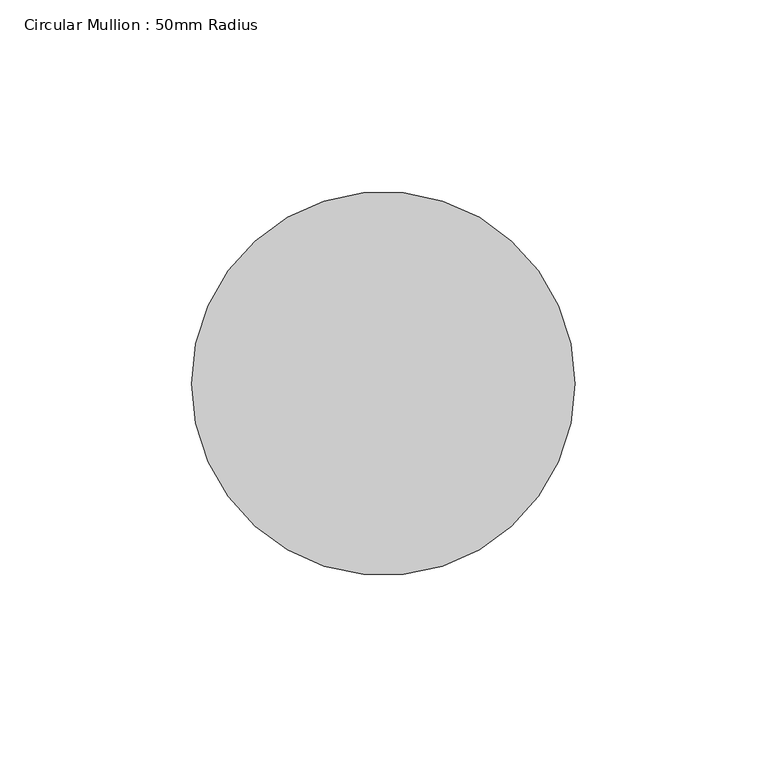
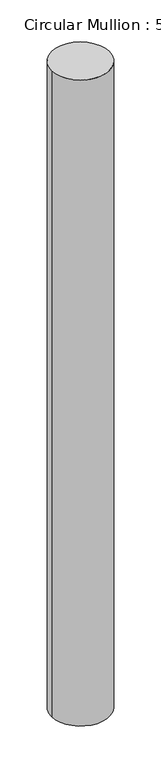
"""IFC4 building model written with IfcOpenShell, lengths in millimetres: member geometry, Circular Mullion : 50mm Radius."""

from ifc_helpers import new_model, si_unit, point, frame, origin, origin_2d, place, context, project, spatial, circle_curve, trimmed, segment, composite_curve, outline, extrude, source, transform, mapped, element, save


def circular_mullion_50mm_radius_26324e7d(model_context):
    return source(origin(), model_context, "Body", "SweptSolid", [
        extrude(outline(composite_curve([segment(trimmed(circle_curve(origin_2d(), 50.0), [point((50.0, 0.0))], [point((-50.0, 0.0))], False, "CARTESIAN"), True, "CONTINUOUS"), segment(trimmed(circle_curve(origin_2d(), 50.0), [point((-50.0, 0.0))], [point((50.0, 0.0))], False, "CARTESIAN"), True, "CONTINUOUS")], self_intersect=False)), frame((0.0, 0.0, -1183.3568083), z_axis=(0.0, 0.0, 1.0), x_axis=(1.0, 0.0, 0.0)), (0.0, 0.0, 1.0), 1183.3568083),
    ])


if __name__ == "__main__":
    model = new_model("IFC4")
    model_context = context("Model", 3, world=origin())
    ifc_project = project(units=[si_unit("LENGTHUNIT", "METRE", prefix="MILLI")], contexts=[model_context])
    site = spatial("IfcSite", under=ifc_project)
    building = spatial("IfcBuilding", under=site)
    placement = place(None, origin())
    circular_mullion_50mm_radius_shape = circular_mullion_50mm_radius_26324e7d(model_context)
    element("IfcMember", 1, ObjectType="Circular Mullion : 50mm Radius", at=placement, inside=building, context=model_context, shape_type="MappedRepresentation", body=[
        mapped(circular_mullion_50mm_radius_shape, transform((0.0, 0.0, 0.0), x_axis=(1.0, 0.0, 0.0), y_axis=(0.0, 1.0, 0.0), z_axis=(0.0, 0.0, 1.0))),
    ])
    save(model, "model.ifc")

# Revit data of these elements
# Type "Circular Mullion : 50mm Radius"
#   built-in parameter 1007350 = 0.164042 (stored number, unit not read)
# Element 1 (IfcMember, "Circular Mullion : 50mm Radius")
#   Materials on its faces: "Aluminium"
# Materials
#   "Aluminium": class "Metal", colour RGB 247 247 247, transparency 0, Description = "Aluminium 6061", Cost = 0
